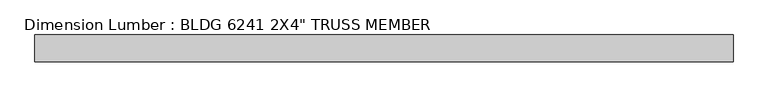
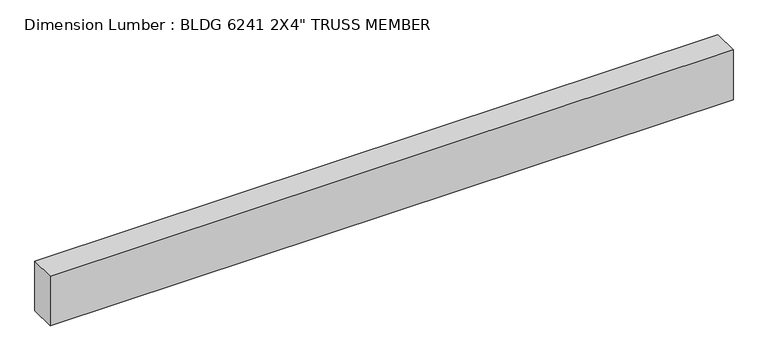
"""IFC4 building model written with IfcOpenShell, lengths in millimetres: beam geometry."""

from ifc_helpers import new_model, si_unit, frame, origin, place, context, project, spatial, polyline, outline, extrude, source, transform, mapped, element, save


def beam_ec20356b(model_context):
    return source(origin(), model_context, "Body", "SweptSolid", [
        extrude(outline(polyline([(660.3999994, 25.4), (660.3999994, -25.4), (-660.3999994, -25.4), (-660.3999994, 25.4), (660.3999994, 25.4)])), frame((0.0, 0.0, -50.8), z_axis=(0.0, 0.0, 1.0), x_axis=(1.0, 0.0, 0.0)), (0.0, 0.0, 1.0), 101.6),
    ])


if __name__ == "__main__":
    model = new_model("IFC4")
    model_context = context("Model", 3, world=origin())
    ifc_project = project(units=[si_unit("LENGTHUNIT", "METRE", prefix="MILLI")], contexts=[model_context])
    site = spatial("IfcSite", under=ifc_project)
    building = spatial("IfcBuilding", under=site)
    placement = place(None, origin())
    beam_shape = beam_ec20356b(model_context)
    element("IfcBeam", 1, ObjectType="Dimension Lumber : BLDG 6241 2X4\" TRUSS MEMBER", at=placement, inside=building, context=model_context, shape_type="MappedRepresentation", body=[
        mapped(beam_shape, transform((0.0, 0.0, 0.0), x_axis=(1.0, 0.0, 0.0), y_axis=(0.0, 1.0, 0.0), z_axis=(0.0, 0.0, 1.0))),
    ])
    save(model, "model.ifc")

# Revit data of these elements
# Type "Dimension Lumber : BLDG 6241 2X4\" TRUSS MEMBER"
#   Assembly Code = "B10"
#   A = 0.273472 SF
#   Length [instance default] = 5' - 0"
#   b = 0' - 2"
#   d = 0' - 4"
#   Structural Material [instance default] = Softwood, Lumber
# Element 1 (IfcBeam, "Dimension Lumber : BLDG 6241 2X4\" TRUSS MEMBER")
#   Materials on its faces: "Softwood, Lumber"
# Materials
#   "Softwood, Lumber": class "Wood", colour RGB 223 192 134, transparency 0, Description = "Pinus Echinata", Cost = 0
